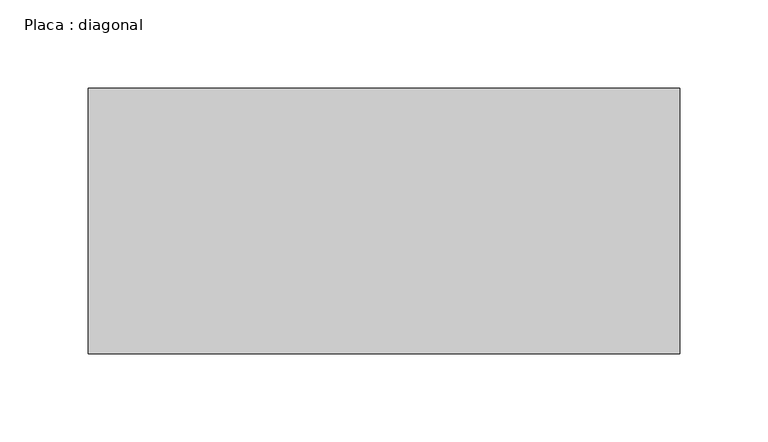
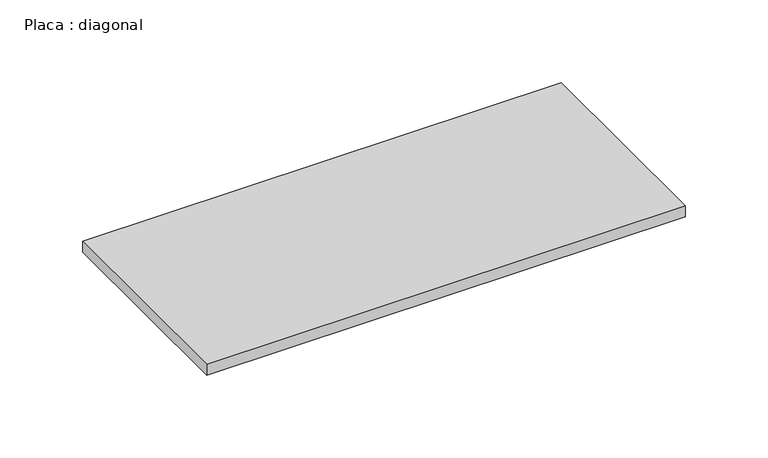
"""IFC4 building model written with IfcOpenShell, lengths in millimetres: beam geometry, Placa : diagonal."""

import ifcopenshell
import ifcopenshell.guid

model = None  # the IFC model being written
_history = None  # IfcOwnerHistory: only IFC2X3 demands one
_inside = {}  # id of a spatial element -> (the spatial element, [elements in it])
_under = {}  # id of a project, library or spatial element -> (it, [spatial elements below it])
_declared = {}  # id of a project -> (the project, [libraries it declares])
_typed = {}  # id of a type object -> (the type object, [elements of that type])
_made_of = {}  # id of a material, layer set ... -> (it, [elements and type objects made of it])


def new_model(schema):
    """Start an empty IFC model of exactly this schema.

    Asked for "IFC4X3", IfcOpenShell would pick the latest addendum, in which some entities
    have other attributes; the version numbers below select the first issue.
    IFC2X3 requires an IfcOwnerHistory on every rooted entity: one is made here for all.
    """
    global model, _history
    if schema == "IFC4X3":
        model = ifcopenshell.file(schema_version=(4, 3, 0, 0))
    else:
        model = ifcopenshell.file(schema=schema)
    _inside.clear()
    _under.clear()
    _declared.clear()
    _typed.clear()
    _made_of.clear()
    _history = None
    if model.schema == "IFC2X3":
        org = make("IfcOrganization", Name="unknown")
        user = make(
            "IfcPersonAndOrganization",
            ThePerson=make("IfcPerson", FamilyName="unknown"),
            TheOrganization=org,
        )
        app = make(
            "IfcApplication",
            ApplicationDeveloper=org,
            Version="unknown",
            ApplicationFullName="unknown",
            ApplicationIdentifier="unknown",
        )
        _history = make(
            "IfcOwnerHistory",
            OwningUser=user,
            OwningApplication=app,
            ChangeAction="ADDED",
            CreationDate=0,
        )
    return model


def make(cls, **values):
    """One entity of the class cls with the attributes given. An attribute that is None is left unset."""
    return model.create_entity(
        cls, **{name: value for name, value in values.items() if value is not None}
    )


def rooted(cls, **values):
    """An entity with a GlobalId (a new one), such as an element, a storey or a relation."""
    return make(cls, GlobalId=ifcopenshell.guid.new(), OwnerHistory=_history, **values)


def si_unit(unit_type, name, prefix=None):
    """IfcSIUnit, for example si_unit("LENGTHUNIT", "METRE", prefix="MILLI")."""
    return make("IfcSIUnit", UnitType=unit_type, Prefix=prefix, Name=name)


def assignment(units):
    """IfcUnitAssignment: the units of a project."""
    return None if units is None else make("IfcUnitAssignment", Units=units)


def point(xyz):
    """IfcCartesianPoint."""
    return None if xyz is None else make("IfcCartesianPoint", Coordinates=xyz)


def direction(xyz):
    """IfcDirection."""
    return None if xyz is None else make("IfcDirection", DirectionRatios=xyz)


def frame(location, z_axis=None, x_axis=None):
    """IfcAxis2Placement3D, a coordinate frame: its origin and axes. An axis left out is left unset."""
    return make(
        "IfcAxis2Placement3D",
        Location=point(location),
        Axis=direction(z_axis),
        RefDirection=direction(x_axis),
    )


def origin():
    """The frame at (0, 0, 0) with its axes left unset."""
    return frame((0.0, 0.0, 0.0))


def place(relative_to, where):
    """IfcLocalPlacement: puts the frame where relative to a parent placement (None: the world)."""
    return make(
        "IfcLocalPlacement", PlacementRelTo=relative_to, RelativePlacement=where
    )


def context(
    kind, dimensions, precision=None, world=None, true_north=None, identifier=None
):
    """IfcGeometricRepresentationContext, for example the 3D "Model" context."""
    return make(
        "IfcGeometricRepresentationContext",
        ContextIdentifier=identifier,
        ContextType=kind,
        CoordinateSpaceDimension=dimensions,
        Precision=precision,
        WorldCoordinateSystem=world,
        TrueNorth=true_north,
    )


def project(units=None, contexts=None):
    """IfcProject with its units and contexts."""
    return rooted(
        "IfcProject",
        Name="project",
        RepresentationContexts=contexts,
        UnitsInContext=assignment(units),
    )


def spatial(cls, under=None, at=None, **own):
    """A site, building, storey or space (cls), placed at a placement, below another one or the project."""
    s = rooted(cls, ObjectPlacement=at, **own)
    if under is not None:
        _under.setdefault(under.id(), (under, []))[1].append(s)
    return s


def polyline(points):
    """IfcPolyline through the points."""
    return make("IfcPolyline", Points=[point(p) for p in points])


def outline(outer, holes=None, kind="AREA"):
    """IfcArbitraryClosedProfileDef: a profile drawn as a closed curve; with holes, ...WithVoids."""
    if holes is None:
        return make("IfcArbitraryClosedProfileDef", ProfileType=kind, OuterCurve=outer)
    return make(
        "IfcArbitraryProfileDefWithVoids",
        ProfileType=kind,
        OuterCurve=outer,
        InnerCurves=holes,
    )


def extrude(swept, where, along, depth):
    """IfcExtrudedAreaSolid: the profile swept, set in the frame where, extruded along a direction by depth."""
    return make(
        "IfcExtrudedAreaSolid",
        SweptArea=swept,
        Position=where,
        ExtrudedDirection=direction(along),
        Depth=depth,
    )


def shape(context_of_items, identifier, shape_type, items):
    """IfcShapeRepresentation: the items that make up one representation, for example the "Body"."""
    return make(
        "IfcShapeRepresentation",
        ContextOfItems=context_of_items,
        RepresentationIdentifier=identifier,
        RepresentationType=shape_type,
        Items=items,
    )


def source(mapping_origin, context_of_items, identifier, shape_type, items):
    """IfcRepresentationMap: a shape defined once, which mapped items show again and again."""
    return make(
        "IfcRepresentationMap",
        MappingOrigin=mapping_origin,
        MappedRepresentation=shape(context_of_items, identifier, shape_type, items),
    )


def transform(
    local_origin,
    x_axis=None,
    y_axis=None,
    z_axis=None,
    scale=None,
    scale2=None,
    scale3=None,
    uniform=True,
):
    """IfcCartesianTransformationOperator3D, or its non-uniform kind. x_axis, y_axis, z_axis: its Axis1, 2, 3."""
    if uniform:
        return make(
            "IfcCartesianTransformationOperator3D",
            Axis1=direction(x_axis),
            Axis2=direction(y_axis),
            LocalOrigin=point(local_origin),
            Scale=scale,
            Axis3=direction(z_axis),
        )
    return make(
        "IfcCartesianTransformationOperator3DnonUniform",
        Axis1=direction(x_axis),
        Axis2=direction(y_axis),
        LocalOrigin=point(local_origin),
        Scale=scale,
        Axis3=direction(z_axis),
        Scale2=scale2,
        Scale3=scale3,
    )


def mapped(mapping_source, mapping_target):
    """IfcMappedItem: shows the shape of a source again, moved by a transform."""
    return make(
        "IfcMappedItem", MappingSource=mapping_source, MappingTarget=mapping_target
    )


def made_of(thing, what):
    """Note that an element or type object is made of a material, layer set ...; save() writes the relation."""
    if what is not None:
        _made_of.setdefault(what.id(), (what, []))[1].append(thing)
    return thing


def element(
    cls,
    number,
    at=None,
    inside=None,
    cuts=None,
    type_object=None,
    material=None,
    context=None,
    identifier="Body",
    shape_type=None,
    held_by="IfcProductDefinitionShape",
    body=None,
    shapes=None,
    **own,
):
    """One element of the class cls, such as IfcWall. Its Tag is "e" and its number.

    at: its placement. inside: the storey or other place that contains it. cuts: it is an
    opening in that element (IfcRelVoidsElement). A single representation is given by context,
    identifier, shape_type and body (its items); several are given by shapes. held_by: the class
    of the entity that holds the representations. save() writes the other relations.
    """
    e = rooted(cls, Tag="e%d" % number, ObjectPlacement=at, **own)
    if body is not None:
        shapes = [shape(context, identifier, shape_type, body)]
    if shapes is not None:
        e.Representation = make(held_by, Representations=shapes)
    if inside is not None:
        _inside.setdefault(inside.id(), (inside, []))[1].append(e)
    if cuts is not None:
        rooted(
            "IfcRelVoidsElement", RelatingBuildingElement=cuts, RelatedOpeningElement=e
        )
    if type_object is not None:
        _typed.setdefault(type_object.id(), (type_object, []))[1].append(e)
    return made_of(e, material)


def aggregate(whole, parts):
    """IfcRelAggregates: a whole, such as a stair, and the parts it consists of."""
    return rooted("IfcRelAggregates", RelatingObject=whole, RelatedObjects=parts)


def save(model, path):
    """Write the relations noted so far, then the file.

    IfcRelAggregates (storeys below a building ...), IfcRelContainedInSpatialStructure (elements
    in a storey), IfcRelDefinesByType, IfcRelAssociatesMaterial and IfcRelDeclares: one each for
    every whole, place, type object, material and project.
    """
    for whole, parts in _under.values():
        aggregate(whole, parts)
    for where, things in _inside.values():
        rooted(
            "IfcRelContainedInSpatialStructure",
            RelatedElements=things,
            RelatingStructure=where,
        )
    for kind, things in _typed.values():
        rooted("IfcRelDefinesByType", RelatedObjects=things, RelatingType=kind)
    for what, things in _made_of.values():
        rooted("IfcRelAssociatesMaterial", RelatedObjects=things, RelatingMaterial=what)
    for by, libraries in _declared.values():
        rooted("IfcRelDeclares", RelatingContext=by, RelatedDefinitions=libraries)
    model.write(path)


def placa_diagonal_4690b74a(model_context):
    return source(origin(), model_context, "Body", "SweptSolid", [
        extrude(outline(polyline([(167.0675389, 75.0), (167.0675389, -75.0), (-167.4240162, -75.0), (-167.4240162, 75.0), (167.0675389, 75.0)])), frame((0.0, 0.0, -4.0), z_axis=(0.0, 0.0, 1.0), x_axis=(1.0, 0.0, 0.0)), (0.0, 0.0, 1.0), 8.0),
    ])


if __name__ == "__main__":
    model = new_model("IFC4")
    model_context = context("Model", 3, world=origin())
    ifc_project = project(units=[si_unit("LENGTHUNIT", "METRE", prefix="MILLI")], contexts=[model_context])
    site = spatial("IfcSite", under=ifc_project)
    building = spatial("IfcBuilding", under=site)
    placement = place(None, origin())
    placa_diagonal_shape = placa_diagonal_4690b74a(model_context)
    element("IfcBeam", 1, ObjectType="Placa : diagonal", at=placement, inside=building, context=model_context, shape_type="MappedRepresentation", body=[
        mapped(placa_diagonal_shape, transform((0.0, 0.0, 0.0), x_axis=(1.0, 0.0, 0.0), y_axis=(0.0, 1.0, 0.0), z_axis=(0.0, 0.0, 1.0))),
    ])
    save(model, "model.ifc")

# Revit data of these elements
# Type "Placa : diagonal"
#   W = 0
#   Length [instance default] = 1.50 m
#   b = 0.15 m
#   d = 0.008 m
#   A = 0 m²
#   Structural Material [instance default] = Aço, 45-345
# Element 1 (IfcBeam, "Placa : diagonal")
#   Materials on its faces: "Aço, 45-345"
# Materials
#   "Aço, 45-345": class "Metal", colour RGB 247 247 247, transparency 0, Description = "Aço 345 MPa", Cost = 0
